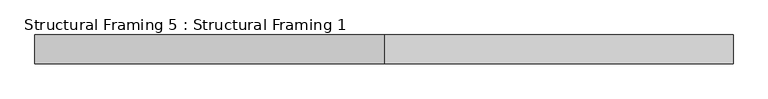
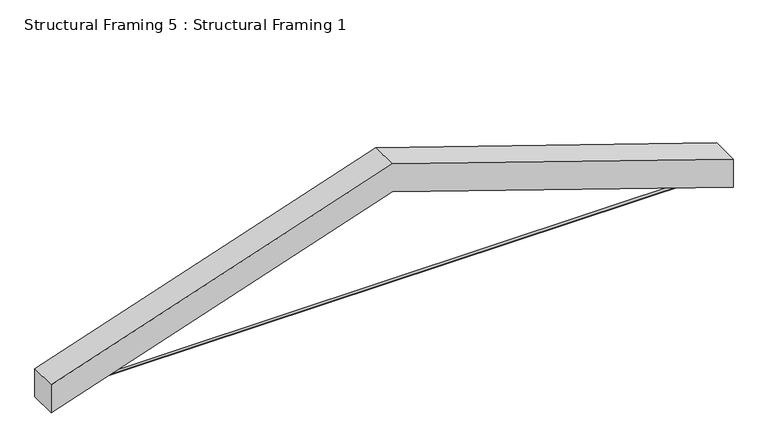
"""IFC4 building model written with IfcOpenShell, lengths in millimetres: beam geometry, Structural Framing 5 : Structural Framing 1."""

from ifc_helpers import new_model, si_unit, point, frame, frame_2d, origin, place, context, project, spatial, polyline, circle_curve, trimmed, segment, composite_curve, outline, extrude, source, transform, mapped, element, save


def structural_framing_5_structural_framing_1_a9d1e016(model_context):
    return source(origin(), model_context, "Body", "SweptSolid", [
        extrude(outline(composite_curve([segment(trimmed(circle_curve(frame_2d((-2265.6884634, 4984.3019529)), 6.35), [point((-2259.3384634, 4984.3019529))], [point((-2272.0384634, 4984.3019529))], False, "CARTESIAN"), True, "CONTINUOUS"), segment(trimmed(circle_curve(frame_2d((-2265.6884634, 4984.3019529)), 6.35), [point((-2272.0384634, 4984.3019529))], [point((-2259.3384634, 4984.3019529))], False, "CARTESIAN"), True, "CONTINUOUS")], self_intersect=False)), frame((19888.9870052, 0.0, 0.0), z_axis=(1.0, 0.0, 0.0), x_axis=(0.0, 1.0, 0.0)), (0.0, 0.0, 1.0), 3111.5),
        extrude(outline(polyline([(5652.475838, 21444.7370052), (5084.8528105, 19749.2870052), (4937.5315162, 19749.2870052), (5505.1545437, 21444.7370052), (4937.5315162, 23140.1870052), (5084.8528105, 23140.1870052), (5652.475838, 21444.7370052)])), frame((0.0, -2335.5384634, 0.0), z_axis=(0.0, 1.0, 0.0), x_axis=(0.0, 0.0, 1.0)), (0.0, 0.0, 1.0), 139.7),
    ])


if __name__ == "__main__":
    model = new_model("IFC4")
    model_context = context("Model", 3, world=origin())
    ifc_project = project(units=[si_unit("LENGTHUNIT", "METRE", prefix="MILLI")], contexts=[model_context])
    site = spatial("IfcSite", under=ifc_project)
    building = spatial("IfcBuilding", under=site)
    placement = place(None, origin())
    structural_framing_5_structural_framing_1_shape = structural_framing_5_structural_framing_1_a9d1e016(model_context)
    element("IfcBeam", 1, ObjectType="Structural Framing 5 : Structural Framing 1", at=placement, inside=building, context=model_context, shape_type="MappedRepresentation", body=[
        mapped(structural_framing_5_structural_framing_1_shape, transform((0.0, 0.0, 0.0), x_axis=(1.0, 0.0, 0.0), y_axis=(0.0, 1.0, 0.0), z_axis=(0.0, 0.0, 1.0))),
    ])
    save(model, "model.ifc")

# Revit data of these elements
# Element 1 (IfcBeam, "Structural Framing 5 : Structural Framing 1")
#   Materials on its faces: "GLULAM TRUSS W/ CUSTOM GUSSET PLATES", "COLLAR TIE: 1/2\" GALV. ROD"
# Materials
#   "GLULAM TRUSS W/ CUSTOM GUSSET PLATES": class "Generic", colour RGB 206 153 90, transparency 0, Cost = 0
#   "COLLAR TIE: 1/2\" GALV. ROD": class "Generic", colour RGB 49 49 49, transparency 0, Cost = 0
